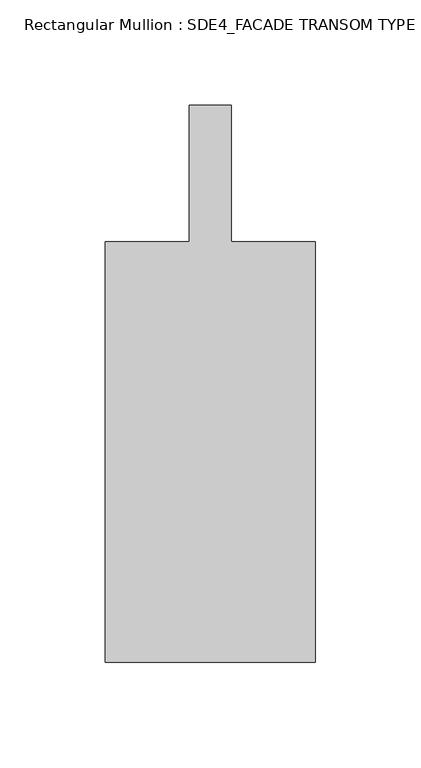
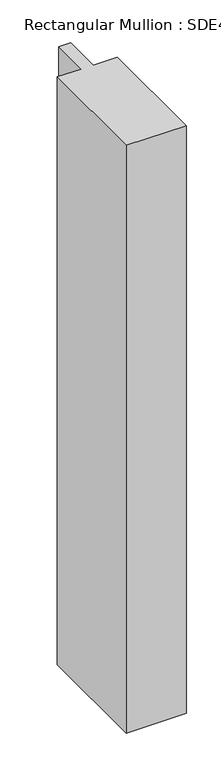
"""IFC4 building model written with IfcOpenShell, lengths in millimetres: member geometry, Rectangular Mullion : SDE4_FACADE TRANSOM TYPE 2."""

import ifcopenshell
import ifcopenshell.guid

model = None  # the IFC model being written
_history = None  # IfcOwnerHistory: only IFC2X3 demands one
_inside = {}  # id of a spatial element -> (the spatial element, [elements in it])
_under = {}  # id of a project, library or spatial element -> (it, [spatial elements below it])
_declared = {}  # id of a project -> (the project, [libraries it declares])
_typed = {}  # id of a type object -> (the type object, [elements of that type])
_made_of = {}  # id of a material, layer set ... -> (it, [elements and type objects made of it])


def new_model(schema):
    """Start an empty IFC model of exactly this schema.

    Asked for "IFC4X3", IfcOpenShell would pick the latest addendum, in which some entities
    have other attributes; the version numbers below select the first issue.
    IFC2X3 requires an IfcOwnerHistory on every rooted entity: one is made here for all.
    """
    global model, _history
    if schema == "IFC4X3":
        model = ifcopenshell.file(schema_version=(4, 3, 0, 0))
    else:
        model = ifcopenshell.file(schema=schema)
    _inside.clear()
    _under.clear()
    _declared.clear()
    _typed.clear()
    _made_of.clear()
    _history = None
    if model.schema == "IFC2X3":
        org = make("IfcOrganization", Name="unknown")
        user = make(
            "IfcPersonAndOrganization",
            ThePerson=make("IfcPerson", FamilyName="unknown"),
            TheOrganization=org,
        )
        app = make(
            "IfcApplication",
            ApplicationDeveloper=org,
            Version="unknown",
            ApplicationFullName="unknown",
            ApplicationIdentifier="unknown",
        )
        _history = make(
            "IfcOwnerHistory",
            OwningUser=user,
            OwningApplication=app,
            ChangeAction="ADDED",
            CreationDate=0,
        )
    return model


def make(cls, **values):
    """One entity of the class cls with the attributes given. An attribute that is None is left unset."""
    return model.create_entity(
        cls, **{name: value for name, value in values.items() if value is not None}
    )


def rooted(cls, **values):
    """An entity with a GlobalId (a new one), such as an element, a storey or a relation."""
    return make(cls, GlobalId=ifcopenshell.guid.new(), OwnerHistory=_history, **values)


def si_unit(unit_type, name, prefix=None):
    """IfcSIUnit, for example si_unit("LENGTHUNIT", "METRE", prefix="MILLI")."""
    return make("IfcSIUnit", UnitType=unit_type, Prefix=prefix, Name=name)


def assignment(units):
    """IfcUnitAssignment: the units of a project."""
    return None if units is None else make("IfcUnitAssignment", Units=units)


def point(xyz):
    """IfcCartesianPoint."""
    return None if xyz is None else make("IfcCartesianPoint", Coordinates=xyz)


def direction(xyz):
    """IfcDirection."""
    return None if xyz is None else make("IfcDirection", DirectionRatios=xyz)


def frame(location, z_axis=None, x_axis=None):
    """IfcAxis2Placement3D, a coordinate frame: its origin and axes. An axis left out is left unset."""
    return make(
        "IfcAxis2Placement3D",
        Location=point(location),
        Axis=direction(z_axis),
        RefDirection=direction(x_axis),
    )


def origin():
    """The frame at (0, 0, 0) with its axes left unset."""
    return frame((0.0, 0.0, 0.0))


def place(relative_to, where):
    """IfcLocalPlacement: puts the frame where relative to a parent placement (None: the world)."""
    return make(
        "IfcLocalPlacement", PlacementRelTo=relative_to, RelativePlacement=where
    )


def context(
    kind, dimensions, precision=None, world=None, true_north=None, identifier=None
):
    """IfcGeometricRepresentationContext, for example the 3D "Model" context."""
    return make(
        "IfcGeometricRepresentationContext",
        ContextIdentifier=identifier,
        ContextType=kind,
        CoordinateSpaceDimension=dimensions,
        Precision=precision,
        WorldCoordinateSystem=world,
        TrueNorth=true_north,
    )


def project(units=None, contexts=None):
    """IfcProject with its units and contexts."""
    return rooted(
        "IfcProject",
        Name="project",
        RepresentationContexts=contexts,
        UnitsInContext=assignment(units),
    )


def spatial(cls, under=None, at=None, **own):
    """A site, building, storey or space (cls), placed at a placement, below another one or the project."""
    s = rooted(cls, ObjectPlacement=at, **own)
    if under is not None:
        _under.setdefault(under.id(), (under, []))[1].append(s)
    return s


def polyline(points):
    """IfcPolyline through the points."""
    return make("IfcPolyline", Points=[point(p) for p in points])


def outline(outer, holes=None, kind="AREA"):
    """IfcArbitraryClosedProfileDef: a profile drawn as a closed curve; with holes, ...WithVoids."""
    if holes is None:
        return make("IfcArbitraryClosedProfileDef", ProfileType=kind, OuterCurve=outer)
    return make(
        "IfcArbitraryProfileDefWithVoids",
        ProfileType=kind,
        OuterCurve=outer,
        InnerCurves=holes,
    )


def extrude(swept, where, along, depth):
    """IfcExtrudedAreaSolid: the profile swept, set in the frame where, extruded along a direction by depth."""
    return make(
        "IfcExtrudedAreaSolid",
        SweptArea=swept,
        Position=where,
        ExtrudedDirection=direction(along),
        Depth=depth,
    )


def shape(context_of_items, identifier, shape_type, items):
    """IfcShapeRepresentation: the items that make up one representation, for example the "Body"."""
    return make(
        "IfcShapeRepresentation",
        ContextOfItems=context_of_items,
        RepresentationIdentifier=identifier,
        RepresentationType=shape_type,
        Items=items,
    )


def source(mapping_origin, context_of_items, identifier, shape_type, items):
    """IfcRepresentationMap: a shape defined once, which mapped items show again and again."""
    return make(
        "IfcRepresentationMap",
        MappingOrigin=mapping_origin,
        MappedRepresentation=shape(context_of_items, identifier, shape_type, items),
    )


def transform(
    local_origin,
    x_axis=None,
    y_axis=None,
    z_axis=None,
    scale=None,
    scale2=None,
    scale3=None,
    uniform=True,
):
    """IfcCartesianTransformationOperator3D, or its non-uniform kind. x_axis, y_axis, z_axis: its Axis1, 2, 3."""
    if uniform:
        return make(
            "IfcCartesianTransformationOperator3D",
            Axis1=direction(x_axis),
            Axis2=direction(y_axis),
            LocalOrigin=point(local_origin),
            Scale=scale,
            Axis3=direction(z_axis),
        )
    return make(
        "IfcCartesianTransformationOperator3DnonUniform",
        Axis1=direction(x_axis),
        Axis2=direction(y_axis),
        LocalOrigin=point(local_origin),
        Scale=scale,
        Axis3=direction(z_axis),
        Scale2=scale2,
        Scale3=scale3,
    )


def mapped(mapping_source, mapping_target):
    """IfcMappedItem: shows the shape of a source again, moved by a transform."""
    return make(
        "IfcMappedItem", MappingSource=mapping_source, MappingTarget=mapping_target
    )


def made_of(thing, what):
    """Note that an element or type object is made of a material, layer set ...; save() writes the relation."""
    if what is not None:
        _made_of.setdefault(what.id(), (what, []))[1].append(thing)
    return thing


def element(
    cls,
    number,
    at=None,
    inside=None,
    cuts=None,
    type_object=None,
    material=None,
    context=None,
    identifier="Body",
    shape_type=None,
    held_by="IfcProductDefinitionShape",
    body=None,
    shapes=None,
    **own,
):
    """One element of the class cls, such as IfcWall. Its Tag is "e" and its number.

    at: its placement. inside: the storey or other place that contains it. cuts: it is an
    opening in that element (IfcRelVoidsElement). A single representation is given by context,
    identifier, shape_type and body (its items); several are given by shapes. held_by: the class
    of the entity that holds the representations. save() writes the other relations.
    """
    e = rooted(cls, Tag="e%d" % number, ObjectPlacement=at, **own)
    if body is not None:
        shapes = [shape(context, identifier, shape_type, body)]
    if shapes is not None:
        e.Representation = make(held_by, Representations=shapes)
    if inside is not None:
        _inside.setdefault(inside.id(), (inside, []))[1].append(e)
    if cuts is not None:
        rooted(
            "IfcRelVoidsElement", RelatingBuildingElement=cuts, RelatedOpeningElement=e
        )
    if type_object is not None:
        _typed.setdefault(type_object.id(), (type_object, []))[1].append(e)
    return made_of(e, material)


def aggregate(whole, parts):
    """IfcRelAggregates: a whole, such as a stair, and the parts it consists of."""
    return rooted("IfcRelAggregates", RelatingObject=whole, RelatedObjects=parts)


def save(model, path):
    """Write the relations noted so far, then the file.

    IfcRelAggregates (storeys below a building ...), IfcRelContainedInSpatialStructure (elements
    in a storey), IfcRelDefinesByType, IfcRelAssociatesMaterial and IfcRelDeclares: one each for
    every whole, place, type object, material and project.
    """
    for whole, parts in _under.values():
        aggregate(whole, parts)
    for where, things in _inside.values():
        rooted(
            "IfcRelContainedInSpatialStructure",
            RelatedElements=things,
            RelatingStructure=where,
        )
    for kind, things in _typed.values():
        rooted("IfcRelDefinesByType", RelatedObjects=things, RelatingType=kind)
    for what, things in _made_of.values():
        rooted("IfcRelAssociatesMaterial", RelatedObjects=things, RelatingMaterial=what)
    for by, libraries in _declared.values():
        rooted("IfcRelDeclares", RelatingContext=by, RelatedDefinitions=libraries)
    model.write(path)


def rectangular_mullion_sde4_facade_transom_type_2_e27847cd(model_context):
    return source(origin(), model_context, "Body", "SweptSolid", [
        extrude(outline(polyline([(50.0, -132.5), (-50.0, -132.5), (-50.0, 67.5), (-10.0, 67.5), (-10.0, 132.5), (10.0, 132.5), (10.0, 67.5), (50.0, 67.5), (50.0, -132.5)])), frame((0.0, 0.0, -1039.9999999), z_axis=(0.0, 0.0, 1.0), x_axis=(1.0, 0.0, 0.0)), (0.0, 0.0, 1.0), 1039.9999999),
    ])


if __name__ == "__main__":
    model = new_model("IFC4")
    model_context = context("Model", 3, world=origin())
    ifc_project = project(units=[si_unit("LENGTHUNIT", "METRE", prefix="MILLI")], contexts=[model_context])
    site = spatial("IfcSite", under=ifc_project)
    building = spatial("IfcBuilding", under=site)
    placement = place(None, origin())
    rectangular_mullion_sde4_facade_transom_type_2_shape = rectangular_mullion_sde4_facade_transom_type_2_e27847cd(model_context)
    element("IfcMember", 1, ObjectType="Rectangular Mullion : SDE4_FACADE TRANSOM TYPE 2", at=placement, inside=building, context=model_context, shape_type="MappedRepresentation", body=[
        mapped(rectangular_mullion_sde4_facade_transom_type_2_shape, transform((0.0, 0.0, 0.0), x_axis=(1.0, 0.0, 0.0), y_axis=(0.0, 1.0, 0.0), z_axis=(0.0, 0.0, 1.0))),
    ])
    save(model, "model.ifc")

# Revit data of these elements
# Type "Rectangular Mullion : SDE4_FACADE TRANSOM TYPE 2"
#   built-in parameter 1007322 = 0.869423 (stored number, unit not read)
#   built-in parameter 1007321 = 0.164042 (stored number, unit not read)
#   built-in parameter 1007320 = 0.164042 (stored number, unit not read)
